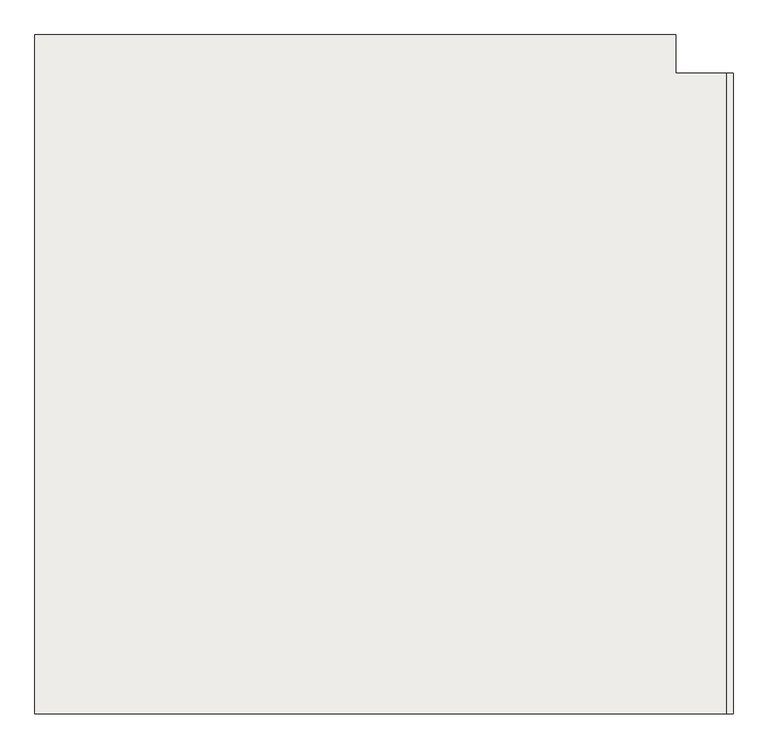
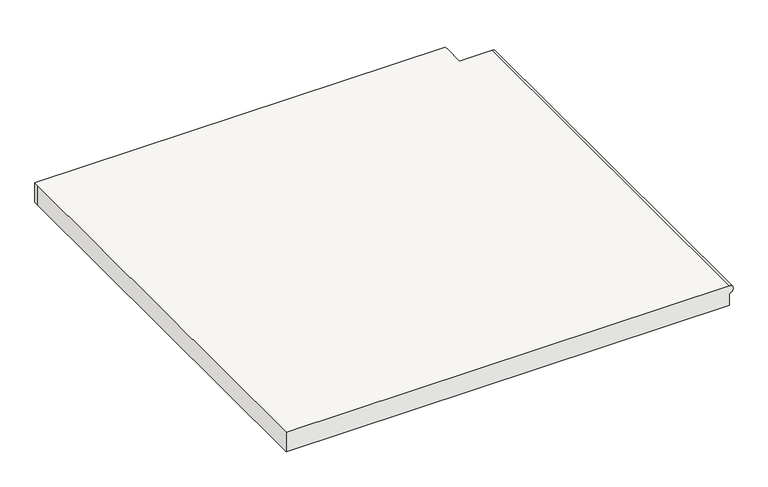
"""IFC4 building model written with IfcOpenShell, lengths in millimetres: slab geometry."""

from ifc_helpers import new_model, si_unit, frame, origin, place, context, project, spatial, circle_curve, source, transform, mapped, element, save
from ifc_brep_helpers import plane_surface, cylinder_surface, advanced_brep


def slab_10a918a9(model_context):
    return source(origin(), model_context, "Body", "AdvancedBrep", [
        advanced_brep(
        [(-2595.8194784, -2645.3813072, 638.8235294), (-2595.8194784, -2645.3813072, 658.8235294), (-2595.8194784, -3645.3813072, 658.8235294), (-2595.8194784, -3645.3813072, 638.8235294), (-2675.5365014, -2645.3813072, 658.8235294), (-2675.5365014, -2595.3813072, 658.8235294), (-2675.5365014, -2585.3813072, 658.8235294), (-3675.5365014, -2585.3813072, 658.8235294), (-3675.5365014, -2595.3813072, 658.8235294), (-3675.5365014, -3645.3813072, 658.8235294), (-2595.8194784, -2645.3813072, 608.8235294), (-2595.8194784, -3645.3813072, 608.8235294), (-3675.5365014, -3645.3813072, 608.8235294), (-3675.5365014, -2595.3813072, 608.8235294), (-3675.5365014, -2585.3813072, 608.8235294), (-2675.5365014, -2585.3813072, 608.8235294), (-2675.5365014, -2595.3813072, 608.8235294), (-2675.5365014, -2645.3813072, 608.8235294)],
        [
            (0, 1, circle_curve(frame((-2595.8194784, -2645.3813072, 648.8235294), z_axis=(0.0, -1.0, 0.0), x_axis=(-1.0, 0.0, 0.0)), 10.0)),
            (1, 2),
            (2, 3, circle_curve(frame((-2595.8194784, -3645.3813072, 648.8235294), z_axis=(0.0, 1.0, 0.0), x_axis=(-1.0, 0.0, 0.0)), 10.0)),
            (3, 0),
            (1, 4),
            (4, 5),
            (5, 6),
            (6, 7),
            (7, 8),
            (8, 9),
            (9, 2),
            (10, 11),
            (11, 12),
            (12, 13),
            (13, 14),
            (14, 15),
            (15, 16),
            (16, 17),
            (17, 10),
            (10, 0),
            (3, 11),
            (17, 4),
            (16, 5),
            (15, 6),
            (14, 7),
            (13, 8),
            (12, 9),
        ],
        [
            cylinder_surface(frame((-2595.8194784, -2645.3813072, 648.8235294), z_axis=(0.0, 1.0, 0.0), x_axis=(-1.0, 0.0, 0.0)), 10.0),
            plane_surface(frame((-2595.8194784, -3645.3813072, 658.8235294), z_axis=(0.0, 0.0, 1.0), x_axis=(0.0, 1.0, 0.0))),
            plane_surface(frame((-2595.8194784, -3645.3813072, 608.8235294), z_axis=(0.0, 0.0, -1.0), x_axis=(0.0, -1.0, 0.0))),
            plane_surface(frame((-2595.8194784, -3645.3813072, 658.8235294), z_axis=(1.0, 0.0, 0.0), x_axis=(0.0, 0.0, -1.0))),
            plane_surface(frame((-2595.8194784, -2645.3813072, 658.8235294), z_axis=(0.0, 1.0, 0.0), x_axis=(0.0, 0.0, -1.0))),
            plane_surface(frame((-2675.5365014, -2645.3813072, 658.8235294), z_axis=(1.0, 0.0, 0.0), x_axis=(0.0, 0.0, -1.0))),
            plane_surface(frame((-2675.5365014, -2595.3813072, 658.8235294), z_axis=(1.0, 0.0, 0.0), x_axis=(0.0, 0.0, -1.0))),
            plane_surface(frame((-2675.5365014, -2585.3813072, 658.8235294), z_axis=(0.0, 1.0, 0.0), x_axis=(0.0, 0.0, -1.0))),
            plane_surface(frame((-3675.5365014, -2585.3813072, 658.8235294), z_axis=(-1.0, 0.0, 0.0), x_axis=(0.0, 0.0, -1.0))),
            plane_surface(frame((-3675.5365014, -2595.3813072, 658.8235294), z_axis=(-1.0, 0.0, 0.0), x_axis=(0.0, 0.0, -1.0))),
            plane_surface(frame((-3675.5365014, -3645.3813072, 658.8235294), z_axis=(0.0, -1.0, 0.0), x_axis=(0.0, 0.0, -1.0))),
        ],
        [
            (0, [[1, 2, 3, 4]]),
            (1, [[5, 6, 7, 8, 9, 10, 11, -2]]),
            (2, [[12, 13, 14, 15, 16, 17, 18, 19]]),
            (3, [[-12, 20, -4, 21]]),
            (4, [[-5, -1, -20, -19, 22]]),
            (5, [[-6, -22, -18, 23]]),
            (6, [[-7, -23, -17, 24]]),
            (7, [[-8, -24, -16, 25]]),
            (8, [[-9, -25, -15, 26]]),
            (9, [[-10, -26, -14, 27]]),
            (10, [[-11, -27, -13, -21, -3]]),
        ],
    ),
    ])


if __name__ == "__main__":
    model = new_model("IFC4")
    model_context = context("Model", 3, world=origin())
    ifc_project = project(units=[si_unit("LENGTHUNIT", "METRE", prefix="MILLI")], contexts=[model_context])
    site = spatial("IfcSite", under=ifc_project)
    building = spatial("IfcBuilding", under=site)
    placement = place(None, origin())
    slab_shape = slab_10a918a9(model_context)
    element("IfcSlab", 1, at=placement, inside=building, context=model_context, shape_type="MappedRepresentation", body=[
        mapped(slab_shape, transform((0.0, 0.0, 0.0), x_axis=(1.0, 0.0, 0.0), y_axis=(0.0, 1.0, 0.0), z_axis=(0.0, 0.0, 1.0))),
    ])
    save(model, "model.ifc")

# Revit data of these elements
# Element 1 (IfcSlab)
#   Materials on its faces: "Oak Flooring"
# Materials
#   "Oak Flooring": class "Wood", colour RGB 212 179 113, transparency 0, Description = "Quercus Rubra", Cost = 0
